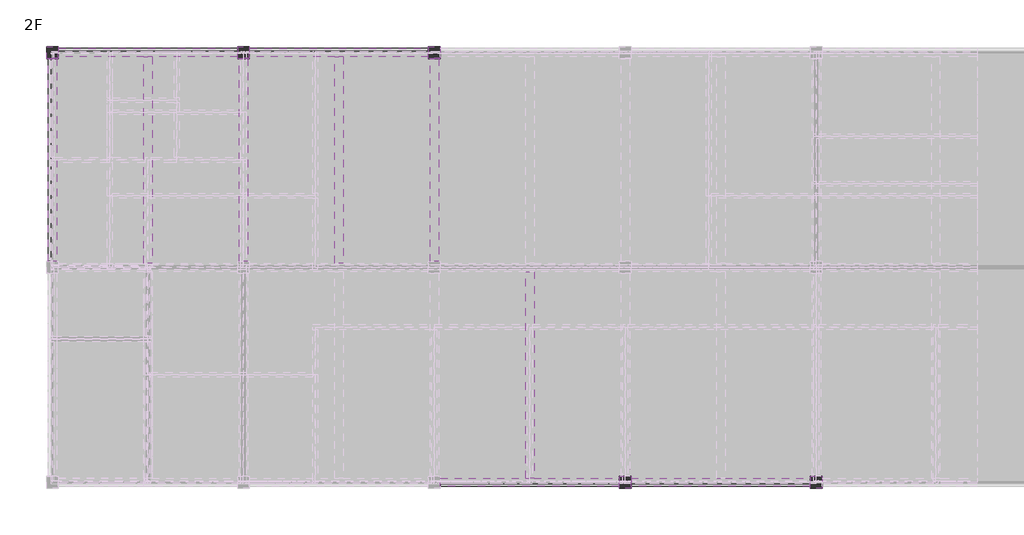
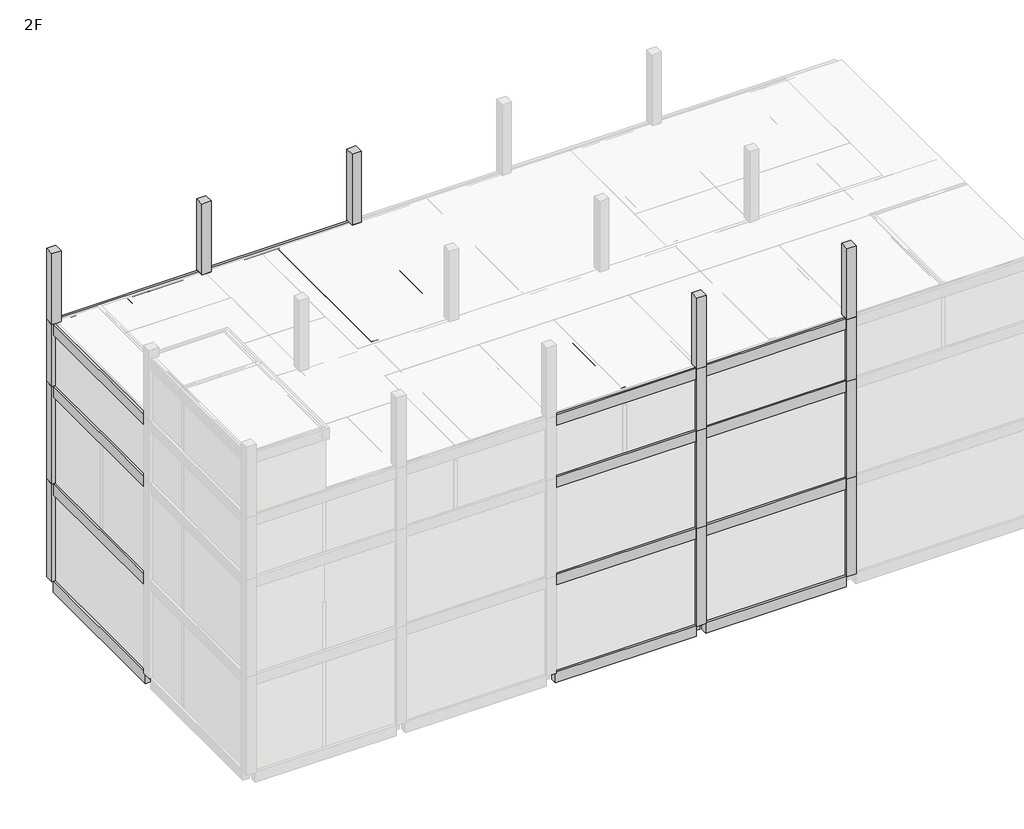
# One storey, part 5 of 7: 42 beams, 20 columns.
"""IFC4 building model written with IfcOpenShell, lengths in millimetres."""

from ifc_helpers import new_model, si_unit, frame, origin, place, context, project, spatial, polyline, outline, extrude, faceted_brep, element, save

model = new_model("IFC4")

# Units and contexts
model_context = context("Model", 3, world=origin())
ifc_project = project(units=[si_unit("LENGTHUNIT", "METRE", prefix="MILLI")], contexts=[model_context])

# Site, building, storey
site = spatial("IfcSite", under=ifc_project)
building = spatial("IfcBuilding", under=site)
storey = spatial("IfcBuildingStorey", under=building, Name="2F", Elevation=3500.0)

# Beams
placement = place(None, origin())
element("IfcBeam", 1, ObjectType="Concrete-Rectangular-Beam : BM111_400x500_RG1", at=placement, inside=storey, context=model_context, shape_type="SweptSolid", body=[
    extrude(outline(polyline([(49284.6521483, 181748.8614395), (49634.6521483, 181748.8614395), (49634.6521483, 173098.8614395), (49284.6521483, 173098.8614395), (49284.6521483, 181748.8614395)])), frame((0.0, 0.0, 2900.0), z_axis=(0.0, 0.0, 1.0), x_axis=(1.0, 0.0, 0.0)), (0.0, 0.0, 1.0), 600.0),
])
element("IfcBeam", 2, ObjectType="Concrete-Rectangular-Beam : BM111_400x500_RG1", at=placement, inside=storey, context=model_context, shape_type="SweptSolid", body=[
    extrude(outline(polyline([(57634.6521483, 173098.8614395), (57284.6521483, 173098.8614395), (57284.6521483, 181748.8614395), (57634.6521483, 181748.8614395), (57634.6521483, 173098.8614395)])), frame((0.0, 0.0, 2900.0), z_axis=(0.0, 0.0, 1.0), x_axis=(1.0, 0.0, 0.0)), (0.0, 0.0, 1.0), 600.0),
])
element("IfcBeam", 3, ObjectType="Concrete-Rectangular-Beam : BM111_400x500_RG1", at=placement, inside=storey, context=model_context, shape_type="SweptSolid", body=[
    extrude(outline(polyline([(65284.6521483, 172748.8614395), (65634.6521483, 172748.8614395), (65634.6521483, 164098.8614395), (65284.6521483, 164098.8614395), (65284.6521483, 172748.8614395)])), frame((0.0, 0.0, 2900.0), z_axis=(0.0, 0.0, 1.0), x_axis=(1.0, 0.0, 0.0)), (0.0, 0.0, 1.0), 600.0),
])
element("IfcBeam", 4, ObjectType="Concrete-Rectangular-Beam : BM111_400x500_RG1", at=placement, inside=storey, context=model_context, shape_type="SweptSolid", body=[
    extrude(outline(polyline([(49284.6521483, 181748.8614395), (49634.6521483, 181748.8614395), (49634.6521483, 173098.8614395), (49284.6521483, 173098.8614395), (49284.6521483, 181748.8614395)])), frame((0.0, 0.0, 8400.0), z_axis=(0.0, 0.0, 1.0), x_axis=(1.0, 0.0, 0.0)), (0.0, 0.0, 1.0), 600.0),
])
element("IfcBeam", 5, ObjectType="Concrete-Rectangular-Beam : BM111_400x500_RG1", at=placement, inside=storey, context=model_context, shape_type="SweptSolid", body=[
    extrude(outline(polyline([(57634.6521483, 173098.8614395), (57284.6521483, 173098.8614395), (57284.6521483, 181748.8614395), (57634.6521483, 181748.8614395), (57634.6521483, 173098.8614395)])), frame((0.0, 0.0, 8400.0), z_axis=(0.0, 0.0, 1.0), x_axis=(1.0, 0.0, 0.0)), (0.0, 0.0, 1.0), 600.0),
])
element("IfcBeam", 6, ObjectType="Concrete-Rectangular-Beam : BM111_400x500_RG1", at=placement, inside=storey, context=model_context, shape_type="SweptSolid", body=[
    extrude(outline(polyline([(65284.6521483, 172748.8614395), (65634.6521483, 172748.8614395), (65634.6521483, 164098.8614395), (65284.6521483, 164098.8614395), (65284.6521483, 172748.8614395)])), frame((0.0, 0.0, 8400.0), z_axis=(0.0, 0.0, 1.0), x_axis=(1.0, 0.0, 0.0)), (0.0, 0.0, 1.0), 600.0),
])
element("IfcBeam", 7, ObjectType="Concrete-Rectangular-Beam : BM111_400x500_RG1", at=placement, inside=storey, context=model_context, shape_type="SweptSolid", body=[
    extrude(outline(polyline([(49284.6521483, 181748.8614395), (49634.6521483, 181748.8614395), (49634.6521483, 173098.8614395), (49284.6521483, 173098.8614395), (49284.6521483, 181748.8614395)])), frame((0.0, 0.0, 13900.0), z_axis=(0.0, 0.0, 1.0), x_axis=(1.0, 0.0, 0.0)), (0.0, 0.0, 1.0), 600.0),
])
element("IfcBeam", 8, ObjectType="Concrete-Rectangular-Beam : BM111_400x500_RG1", at=placement, inside=storey, context=model_context, shape_type="SweptSolid", body=[
    extrude(outline(polyline([(57634.6521483, 173098.8614395), (57284.6521483, 173098.8614395), (57284.6521483, 181748.8614395), (57634.6521483, 181748.8614395), (57634.6521483, 173098.8614395)])), frame((0.0, 0.0, 13900.0), z_axis=(0.0, 0.0, 1.0), x_axis=(1.0, 0.0, 0.0)), (0.0, 0.0, 1.0), 600.0),
])
element("IfcBeam", 9, ObjectType="Concrete-Rectangular-Beam : BM111_400x500_RG1", at=placement, inside=storey, context=model_context, shape_type="SweptSolid", body=[
    extrude(outline(polyline([(65284.6521483, 172748.8614395), (65634.6521483, 172748.8614395), (65634.6521483, 164098.8614395), (65284.6521483, 164098.8614395), (65284.6521483, 172748.8614395)])), frame((0.0, 0.0, 13900.0), z_axis=(0.0, 0.0, 1.0), x_axis=(1.0, 0.0, 0.0)), (0.0, 0.0, 1.0), 600.0),
])
element("IfcBeam", 10, ObjectType="Concrete-Rectangular-Beam : BM111_400x500_RG1", at=placement, inside=storey, context=model_context, shape_type="SweptSolid", body=[
    extrude(outline(polyline([(49284.6521483, 181748.8614395), (49634.6521483, 181748.8614395), (49634.6521483, 173098.8614395), (49284.6521483, 173098.8614395), (49284.6521483, 181748.8614395)])), frame((0.0, 0.0, 17400.0), z_axis=(0.0, 0.0, 1.0), x_axis=(1.0, 0.0, 0.0)), (0.0, 0.0, 1.0), 600.0),
])
element("IfcBeam", 11, ObjectType="Concrete-Rectangular-Beam : BM111_400x500_RG1", at=placement, inside=storey, context=model_context, shape_type="SweptSolid", body=[
    extrude(outline(polyline([(57634.6521483, 173098.8614395), (57284.6521483, 173098.8614395), (57284.6521483, 181748.8614395), (57634.6521483, 181748.8614395), (57634.6521483, 173098.8614395)])), frame((0.0, 0.0, 17400.0), z_axis=(0.0, 0.0, 1.0), x_axis=(1.0, 0.0, 0.0)), (0.0, 0.0, 1.0), 600.0),
])
element("IfcBeam", 12, ObjectType="Concrete-Rectangular-Beam : BM111_400x500_RG1", at=placement, inside=storey, context=model_context, shape_type="SweptSolid", body=[
    extrude(outline(polyline([(65284.6521483, 172748.8614395), (65634.6521483, 172748.8614395), (65634.6521483, 164098.8614395), (65284.6521483, 164098.8614395), (65284.6521483, 172748.8614395)])), frame((0.0, 0.0, 17400.0), z_axis=(0.0, 0.0, 1.0), x_axis=(1.0, 0.0, 0.0)), (0.0, 0.0, 1.0), 600.0),
])
element("IfcBeam", 13, ObjectType="Concrete-Rectangular-Beam : BM111_400x500_RG1", at=placement, inside=storey, context=model_context, shape_type="Brep", body=[
    faceted_brep([(45709.6521483, 182098.8614395, 3500.0), (45709.6521483, 181748.8614395, 3500.0), (49284.6521483, 181748.8614395, 3500.0), (49634.6521483, 181748.8614395, 3500.0), (53209.6521483, 181748.8614395, 3500.0), (53209.6521483, 182098.8614395, 3500.0), (45709.6521483, 181748.8614395, 2900.0), (49284.6521483, 181748.8614395, 2900.0), (49634.6521483, 181748.8614395, 2900.0), (53209.6521483, 181748.8614395, 2900.0), (45709.6521483, 182098.8614395, 2900.0), (53209.6521483, 182098.8614395, 2900.0)], [[[0, 1, 2, 3, 4, 5]], [[1, 6, 7, 8, 9, 4, 3, 2]], [[6, 10, 11, 9, 8, 7]], [[10, 0, 5, 11]], [[1, 0, 10, 6]], [[5, 4, 9, 11]]]),
])
element("IfcBeam", 14, ObjectType="Concrete-Rectangular-Beam : BM111_400x500_RG1", at=placement, inside=storey, context=model_context, shape_type="Brep", body=[
    faceted_brep([(53709.6521483, 182098.8614395, 3500.0), (53709.6521483, 181748.8614395, 3500.0), (57284.6521483, 181748.8614395, 3500.0), (57634.6521483, 181748.8614395, 3500.0), (61209.6521483, 181748.8614395, 3500.0), (61209.6521483, 182098.8614395, 3500.0), (53709.6521483, 181748.8614395, 2900.0), (57284.6521483, 181748.8614395, 2900.0), (57634.6521483, 181748.8614395, 2900.0), (61209.6521483, 181748.8614395, 2900.0), (53709.6521483, 182098.8614395, 2900.0), (61209.6521483, 182098.8614395, 2900.0)], [[[0, 1, 2, 3, 4, 5]], [[1, 6, 7, 8, 9, 4, 3, 2]], [[6, 10, 11, 9, 8, 7]], [[10, 0, 5, 11]], [[1, 0, 10, 6]], [[5, 4, 9, 11]]]),
])
element("IfcBeam", 15, ObjectType="Concrete-Rectangular-Beam : BM111_400x500_RG1", at=placement, inside=storey, context=model_context, shape_type="Brep", body=[
    faceted_brep([(61709.6521483, 164098.8614395, 3500.0), (61709.6521483, 163748.8614395, 3500.0), (69209.6521483, 163748.8614395, 3500.0), (69209.6521483, 164098.8614395, 3500.0), (65634.6521483, 164098.8614395, 3500.0), (65284.6521483, 164098.8614395, 3500.0), (61709.6521483, 163748.8614395, 2900.0), (69209.6521483, 163748.8614395, 2900.0), (61709.6521483, 164098.8614395, 2900.0), (65284.6521483, 164098.8614395, 2900.0), (65634.6521483, 164098.8614395, 2900.0), (69209.6521483, 164098.8614395, 2900.0)], [[[0, 1, 2, 3, 4, 5]], [[1, 6, 7, 2]], [[6, 8, 9, 10, 11, 7]], [[8, 0, 5, 4, 3, 11, 10, 9]], [[1, 0, 8, 6]], [[3, 2, 7, 11]]]),
])
element("IfcBeam", 16, ObjectType="Concrete-Rectangular-Beam : BM111_400x500_RG1", at=placement, inside=storey, context=model_context, shape_type="Brep", body=[
    faceted_brep([(69709.6521483, 164098.8614395, 3500.0), (69709.6521483, 163748.8614395, 3500.0), (77209.6521483, 163748.8614395, 3500.0), (77209.6521483, 164098.8614395, 3500.0), (73634.6521483, 164098.8614395, 3500.0), (73284.6521483, 164098.8614395, 3500.0), (69709.6521483, 163748.8614395, 2900.0), (77209.6521483, 163748.8614395, 2900.0), (69709.6521483, 164098.8614395, 2900.0), (73284.6521483, 164098.8614395, 2900.0), (73634.6521483, 164098.8614395, 2900.0), (77209.6521483, 164098.8614395, 2900.0)], [[[0, 1, 2, 3, 4, 5]], [[1, 6, 7, 2]], [[6, 8, 9, 10, 11, 7]], [[8, 0, 5, 4, 3, 11, 10, 9]], [[1, 0, 8, 6]], [[3, 2, 7, 11]]]),
])
element("IfcBeam", 17, ObjectType="Concrete-Rectangular-Beam : BM111_400x500_RG1", at=placement, inside=storey, context=model_context, shape_type="Brep", body=[
    faceted_brep([(45709.6521483, 182098.8614395, 9000.0), (45709.6521483, 181748.8614395, 9000.0), (49284.6521483, 181748.8614395, 9000.0), (49634.6521483, 181748.8614395, 9000.0), (53209.6521483, 181748.8614395, 9000.0), (53209.6521483, 182098.8614395, 9000.0), (45709.6521483, 181748.8614395, 8400.0), (49284.6521483, 181748.8614395, 8400.0), (49634.6521483, 181748.8614395, 8400.0), (53209.6521483, 181748.8614395, 8400.0), (45709.6521483, 182098.8614395, 8400.0), (53209.6521483, 182098.8614395, 8400.0)], [[[0, 1, 2, 3, 4, 5]], [[1, 6, 7, 8, 9, 4, 3, 2]], [[6, 10, 11, 9, 8, 7]], [[10, 0, 5, 11]], [[1, 0, 10, 6]], [[5, 4, 9, 11]]]),
])
element("IfcBeam", 18, ObjectType="Concrete-Rectangular-Beam : BM111_400x500_RG1", at=placement, inside=storey, context=model_context, shape_type="Brep", body=[
    faceted_brep([(53709.6521483, 182098.8614395, 9000.0), (53709.6521483, 181748.8614395, 9000.0), (57284.6521483, 181748.8614395, 9000.0), (57634.6521483, 181748.8614395, 9000.0), (61209.6521483, 181748.8614395, 9000.0), (61209.6521483, 182098.8614395, 9000.0), (53709.6521483, 181748.8614395, 8400.0), (57284.6521483, 181748.8614395, 8400.0), (57634.6521483, 181748.8614395, 8400.0), (61209.6521483, 181748.8614395, 8400.0), (53709.6521483, 182098.8614395, 8400.0), (61209.6521483, 182098.8614395, 8400.0)], [[[0, 1, 2, 3, 4, 5]], [[1, 6, 7, 8, 9, 4, 3, 2]], [[6, 10, 11, 9, 8, 7]], [[10, 0, 5, 11]], [[1, 0, 10, 6]], [[5, 4, 9, 11]]]),
])
element("IfcBeam", 19, ObjectType="Concrete-Rectangular-Beam : BM111_400x500_RG1", at=placement, inside=storey, context=model_context, shape_type="Brep", body=[
    faceted_brep([(61709.6521483, 164098.8614395, 9000.0), (61709.6521483, 163748.8614395, 9000.0), (69209.6521483, 163748.8614395, 9000.0), (69209.6521483, 164098.8614395, 9000.0), (65634.6521483, 164098.8614395, 9000.0), (65284.6521483, 164098.8614395, 9000.0), (61709.6521483, 163748.8614395, 8400.0), (69209.6521483, 163748.8614395, 8400.0), (61709.6521483, 164098.8614395, 8400.0), (65284.6521483, 164098.8614395, 8400.0), (65634.6521483, 164098.8614395, 8400.0), (69209.6521483, 164098.8614395, 8400.0)], [[[0, 1, 2, 3, 4, 5]], [[1, 6, 7, 2]], [[6, 8, 9, 10, 11, 7]], [[8, 0, 5, 4, 3, 11, 10, 9]], [[1, 0, 8, 6]], [[3, 2, 7, 11]]]),
])
element("IfcBeam", 20, ObjectType="Concrete-Rectangular-Beam : BM111_400x500_RG1", at=placement, inside=storey, context=model_context, shape_type="Brep", body=[
    faceted_brep([(69709.6521483, 164098.8614395, 9000.0), (69709.6521483, 163748.8614395, 9000.0), (77209.6521483, 163748.8614395, 9000.0), (77209.6521483, 164098.8614395, 9000.0), (73634.6521483, 164098.8614395, 9000.0), (73284.6521483, 164098.8614395, 9000.0), (69709.6521483, 163748.8614395, 8400.0), (77209.6521483, 163748.8614395, 8400.0), (69709.6521483, 164098.8614395, 8400.0), (73284.6521483, 164098.8614395, 8400.0), (73634.6521483, 164098.8614395, 8400.0), (77209.6521483, 164098.8614395, 8400.0)], [[[0, 1, 2, 3, 4, 5]], [[1, 6, 7, 2]], [[6, 8, 9, 10, 11, 7]], [[8, 0, 5, 4, 3, 11, 10, 9]], [[1, 0, 8, 6]], [[3, 2, 7, 11]]]),
])
element("IfcBeam", 21, ObjectType="Concrete-Rectangular-Beam : BM111_400x500_RG1", at=placement, inside=storey, context=model_context, shape_type="Brep", body=[
    faceted_brep([(45709.6521483, 182098.8614395, 14500.0), (45709.6521483, 181748.8614395, 14500.0), (49284.6521483, 181748.8614395, 14500.0), (49634.6521483, 181748.8614395, 14500.0), (53209.6521483, 181748.8614395, 14500.0), (53209.6521483, 182098.8614395, 14500.0), (45709.6521483, 181748.8614395, 13900.0), (49284.6521483, 181748.8614395, 13900.0), (49634.6521483, 181748.8614395, 13900.0), (53209.6521483, 181748.8614395, 13900.0), (45709.6521483, 182098.8614395, 13900.0), (53209.6521483, 182098.8614395, 13900.0)], [[[0, 1, 2, 3, 4, 5]], [[1, 6, 7, 8, 9, 4, 3, 2]], [[6, 10, 11, 9, 8, 7]], [[10, 0, 5, 11]], [[1, 0, 10, 6]], [[5, 4, 9, 11]]]),
])
element("IfcBeam", 22, ObjectType="Concrete-Rectangular-Beam : BM111_400x500_RG1", at=placement, inside=storey, context=model_context, shape_type="Brep", body=[
    faceted_brep([(53709.6521483, 182098.8614395, 14500.0), (53709.6521483, 181748.8614395, 14500.0), (57284.6521483, 181748.8614395, 14500.0), (57634.6521483, 181748.8614395, 14500.0), (61209.6521483, 181748.8614395, 14500.0), (61209.6521483, 182098.8614395, 14500.0), (53709.6521483, 181748.8614395, 13900.0), (57284.6521483, 181748.8614395, 13900.0), (57634.6521483, 181748.8614395, 13900.0), (61209.6521483, 181748.8614395, 13900.0), (53709.6521483, 182098.8614395, 13900.0), (61209.6521483, 182098.8614395, 13900.0)], [[[0, 1, 2, 3, 4, 5]], [[1, 6, 7, 8, 9, 4, 3, 2]], [[6, 10, 11, 9, 8, 7]], [[10, 0, 5, 11]], [[1, 0, 10, 6]], [[5, 4, 9, 11]]]),
])
element("IfcBeam", 23, ObjectType="Concrete-Rectangular-Beam : BM111_400x500_RG1", at=placement, inside=storey, context=model_context, shape_type="Brep", body=[
    faceted_brep([(61709.6521483, 164098.8614395, 14500.0), (61709.6521483, 163748.8614395, 14500.0), (69209.6521483, 163748.8614395, 14500.0), (69209.6521483, 164098.8614395, 14500.0), (65634.6521483, 164098.8614395, 14500.0), (65284.6521483, 164098.8614395, 14500.0), (61709.6521483, 163748.8614395, 13900.0), (69209.6521483, 163748.8614395, 13900.0), (61709.6521483, 164098.8614395, 13900.0), (65284.6521483, 164098.8614395, 13900.0), (65634.6521483, 164098.8614395, 13900.0), (69209.6521483, 164098.8614395, 13900.0)], [[[0, 1, 2, 3, 4, 5]], [[1, 6, 7, 2]], [[6, 8, 9, 10, 11, 7]], [[8, 0, 5, 4, 3, 11, 10, 9]], [[1, 0, 8, 6]], [[3, 2, 7, 11]]]),
])
element("IfcBeam", 24, ObjectType="Concrete-Rectangular-Beam : BM111_400x500_RG1", at=placement, inside=storey, context=model_context, shape_type="Brep", body=[
    faceted_brep([(69709.6521483, 164098.8614395, 14500.0), (69709.6521483, 163748.8614395, 14500.0), (77209.6521483, 163748.8614395, 14500.0), (77209.6521483, 164098.8614395, 14500.0), (73634.6521483, 164098.8614395, 14500.0), (73284.6521483, 164098.8614395, 14500.0), (69709.6521483, 163748.8614395, 13900.0), (77209.6521483, 163748.8614395, 13900.0), (69709.6521483, 164098.8614395, 13900.0), (73284.6521483, 164098.8614395, 13900.0), (73634.6521483, 164098.8614395, 13900.0), (77209.6521483, 164098.8614395, 13900.0)], [[[0, 1, 2, 3, 4, 5]], [[1, 6, 7, 2]], [[6, 8, 9, 10, 11, 7]], [[8, 0, 5, 4, 3, 11, 10, 9]], [[1, 0, 8, 6]], [[3, 2, 7, 11]]]),
])
element("IfcBeam", 25, ObjectType="Concrete-Rectangular-Beam : BM111_400x500_RG1", at=placement, inside=storey, context=model_context, shape_type="Brep", body=[
    faceted_brep([(45709.6521483, 182098.8614395, 18000.0), (45709.6521483, 181748.8614395, 18000.0), (49284.6521483, 181748.8614395, 18000.0), (49634.6521483, 181748.8614395, 18000.0), (53209.6521483, 181748.8614395, 18000.0), (53209.6521483, 182098.8614395, 18000.0), (45709.6521483, 181748.8614395, 17400.0), (49284.6521483, 181748.8614395, 17400.0), (49634.6521483, 181748.8614395, 17400.0), (53209.6521483, 181748.8614395, 17400.0), (45709.6521483, 182098.8614395, 17400.0), (53209.6521483, 182098.8614395, 17400.0)], [[[0, 1, 2, 3, 4, 5]], [[1, 6, 7, 8, 9, 4, 3, 2]], [[6, 10, 11, 9, 8, 7]], [[10, 0, 5, 11]], [[1, 0, 10, 6]], [[5, 4, 9, 11]]]),
])
element("IfcBeam", 26, ObjectType="Concrete-Rectangular-Beam : BM111_400x500_RG1", at=placement, inside=storey, context=model_context, shape_type="Brep", body=[
    faceted_brep([(53709.6521483, 182098.8614395, 18000.0), (53709.6521483, 181748.8614395, 18000.0), (57284.6521483, 181748.8614395, 18000.0), (57634.6521483, 181748.8614395, 18000.0), (61209.6521483, 181748.8614395, 18000.0), (61209.6521483, 182098.8614395, 18000.0), (53709.6521483, 181748.8614395, 17400.0), (57284.6521483, 181748.8614395, 17400.0), (57634.6521483, 181748.8614395, 17400.0), (61209.6521483, 181748.8614395, 17400.0), (53709.6521483, 182098.8614395, 17400.0), (61209.6521483, 182098.8614395, 17400.0)], [[[0, 1, 2, 3, 4, 5]], [[1, 6, 7, 8, 9, 4, 3, 2]], [[6, 10, 11, 9, 8, 7]], [[10, 0, 5, 11]], [[1, 0, 10, 6]], [[5, 4, 9, 11]]]),
])
element("IfcBeam", 27, ObjectType="Concrete-Rectangular-Beam : BM111_400x500_RG1", at=placement, inside=storey, context=model_context, shape_type="Brep", body=[
    faceted_brep([(61709.6521483, 164098.8614395, 18000.0), (61709.6521483, 163748.8614395, 18000.0), (69209.6521483, 163748.8614395, 18000.0), (69209.6521483, 164098.8614395, 18000.0), (65634.6521483, 164098.8614395, 18000.0), (65284.6521483, 164098.8614395, 18000.0), (61709.6521483, 163748.8614395, 17400.0), (69209.6521483, 163748.8614395, 17400.0), (61709.6521483, 164098.8614395, 17400.0), (65284.6521483, 164098.8614395, 17400.0), (65634.6521483, 164098.8614395, 17400.0), (69209.6521483, 164098.8614395, 17400.0)], [[[0, 1, 2, 3, 4, 5]], [[1, 6, 7, 2]], [[6, 8, 9, 10, 11, 7]], [[8, 0, 5, 4, 3, 11, 10, 9]], [[1, 0, 8, 6]], [[3, 2, 7, 11]]]),
])
element("IfcBeam", 28, ObjectType="Concrete-Rectangular-Beam : BM111_400x500_RG1", at=placement, inside=storey, context=model_context, shape_type="Brep", body=[
    faceted_brep([(69709.6521483, 164098.8614395, 18000.0), (69709.6521483, 163748.8614395, 18000.0), (77209.6521483, 163748.8614395, 18000.0), (77209.6521483, 164098.8614395, 18000.0), (73634.6521483, 164098.8614395, 18000.0), (73284.6521483, 164098.8614395, 18000.0), (69709.6521483, 163748.8614395, 17400.0), (77209.6521483, 163748.8614395, 17400.0), (69709.6521483, 164098.8614395, 17400.0), (73284.6521483, 164098.8614395, 17400.0), (73634.6521483, 164098.8614395, 17400.0), (77209.6521483, 164098.8614395, 17400.0)], [[[0, 1, 2, 3, 4, 5]], [[1, 6, 7, 2]], [[6, 8, 9, 10, 11, 7]], [[8, 0, 5, 4, 3, 11, 10, 9]], [[1, 0, 8, 6]], [[3, 2, 7, 11]]]),
])
element("IfcBeam", 29, ObjectType="Concrete-Rectangular-Beam : BM111_400x500_RG1", at=placement, inside=storey, context=model_context, shape_type="SweptSolid", body=[
    extrude(outline(polyline([(45284.6521483, 181673.8614395), (45634.6521483, 181673.8614395), (45634.6521483, 173173.8614395), (45284.6521483, 173173.8614395), (45284.6521483, 181673.8614395)])), frame((0.0, 0.0, 2900.0), z_axis=(0.0, 0.0, 1.0), x_axis=(1.0, 0.0, 0.0)), (0.0, 0.0, 1.0), 600.0),
])
element("IfcBeam", 30, ObjectType="Concrete-Rectangular-Beam : BM111_400x500_RG1", at=placement, inside=storey, context=model_context, shape_type="SweptSolid", body=[
    extrude(outline(polyline([(53284.6521483, 181673.8614395), (53634.6521483, 181673.8614395), (53634.6521483, 173173.8614395), (53284.6521483, 173173.8614395), (53284.6521483, 181673.8614395)])), frame((0.0, 0.0, 2900.0), z_axis=(0.0, 0.0, 1.0), x_axis=(1.0, 0.0, 0.0)), (0.0, 0.0, 1.0), 600.0),
])
element("IfcBeam", 31, ObjectType="Concrete-Rectangular-Beam : BM111_400x500_RG1", at=placement, inside=storey, context=model_context, shape_type="SweptSolid", body=[
    extrude(outline(polyline([(61284.6521483, 181673.8614395), (61634.6521483, 181673.8614395), (61634.6521483, 173173.8614395), (61284.6521483, 173173.8614395), (61284.6521483, 181673.8614395)])), frame((0.0, 0.0, 2900.0), z_axis=(0.0, 0.0, 1.0), x_axis=(1.0, 0.0, 0.0)), (0.0, 0.0, 1.0), 600.0),
])
element("IfcBeam", 32, ObjectType="Concrete-Rectangular-Beam : BM111_400x500_RG1", at=placement, inside=storey, context=model_context, shape_type="SweptSolid", body=[
    extrude(outline(polyline([(69284.6521483, 172673.8614395), (69634.6521483, 172673.8614395), (69634.6521483, 164173.8614395), (69284.6521483, 164173.8614395), (69284.6521483, 172673.8614395)])), frame((0.0, 0.0, 2900.0), z_axis=(0.0, 0.0, 1.0), x_axis=(1.0, 0.0, 0.0)), (0.0, 0.0, 1.0), 600.0),
])
element("IfcBeam", 33, ObjectType="Concrete-Rectangular-Beam : BM111_400x500_RG1", at=placement, inside=storey, context=model_context, shape_type="SweptSolid", body=[
    extrude(outline(polyline([(45284.6521483, 181673.8614395), (45634.6521483, 181673.8614395), (45634.6521483, 173173.8614395), (45284.6521483, 173173.8614395), (45284.6521483, 181673.8614395)])), frame((0.0, 0.0, 8400.0), z_axis=(0.0, 0.0, 1.0), x_axis=(1.0, 0.0, 0.0)), (0.0, 0.0, 1.0), 600.0),
])
element("IfcBeam", 34, ObjectType="Concrete-Rectangular-Beam : BM111_400x500_RG1", at=placement, inside=storey, context=model_context, shape_type="SweptSolid", body=[
    extrude(outline(polyline([(53284.6521483, 181673.8614395), (53634.6521483, 181673.8614395), (53634.6521483, 173173.8614395), (53284.6521483, 173173.8614395), (53284.6521483, 181673.8614395)])), frame((0.0, 0.0, 8400.0), z_axis=(0.0, 0.0, 1.0), x_axis=(1.0, 0.0, 0.0)), (0.0, 0.0, 1.0), 600.0),
])
element("IfcBeam", 35, ObjectType="Concrete-Rectangular-Beam : BM111_400x500_RG1", at=placement, inside=storey, context=model_context, shape_type="SweptSolid", body=[
    extrude(outline(polyline([(61284.6521483, 181673.8614395), (61634.6521483, 181673.8614395), (61634.6521483, 173173.8614395), (61284.6521483, 173173.8614395), (61284.6521483, 181673.8614395)])), frame((0.0, 0.0, 8400.0), z_axis=(0.0, 0.0, 1.0), x_axis=(1.0, 0.0, 0.0)), (0.0, 0.0, 1.0), 600.0),
])
element("IfcBeam", 36, ObjectType="Concrete-Rectangular-Beam : BM111_400x500_RG1", at=placement, inside=storey, context=model_context, shape_type="SweptSolid", body=[
    extrude(outline(polyline([(69284.6521483, 172673.8614395), (69634.6521483, 172673.8614395), (69634.6521483, 164173.8614395), (69284.6521483, 164173.8614395), (69284.6521483, 172673.8614395)])), frame((0.0, 0.0, 8400.0), z_axis=(0.0, 0.0, 1.0), x_axis=(1.0, 0.0, 0.0)), (0.0, 0.0, 1.0), 600.0),
])
element("IfcBeam", 37, ObjectType="Concrete-Rectangular-Beam : BM111_400x500_RG1", at=placement, inside=storey, context=model_context, shape_type="SweptSolid", body=[
    extrude(outline(polyline([(45284.6521483, 181673.8614395), (45634.6521483, 181673.8614395), (45634.6521483, 173173.8614395), (45284.6521483, 173173.8614395), (45284.6521483, 181673.8614395)])), frame((0.0, 0.0, 13900.0), z_axis=(0.0, 0.0, 1.0), x_axis=(1.0, 0.0, 0.0)), (0.0, 0.0, 1.0), 600.0),
])
element("IfcBeam", 38, ObjectType="Concrete-Rectangular-Beam : BM111_400x500_RG1", at=placement, inside=storey, context=model_context, shape_type="SweptSolid", body=[
    extrude(outline(polyline([(53284.6521483, 181673.8614395), (53634.6521483, 181673.8614395), (53634.6521483, 173173.8614395), (53284.6521483, 173173.8614395), (53284.6521483, 181673.8614395)])), frame((0.0, 0.0, 13900.0), z_axis=(0.0, 0.0, 1.0), x_axis=(1.0, 0.0, 0.0)), (0.0, 0.0, 1.0), 600.0),
])
element("IfcBeam", 39, ObjectType="Concrete-Rectangular-Beam : BM111_400x500_RG1", at=placement, inside=storey, context=model_context, shape_type="SweptSolid", body=[
    extrude(outline(polyline([(61284.6521483, 181673.8614395), (61634.6521483, 181673.8614395), (61634.6521483, 173173.8614395), (61284.6521483, 173173.8614395), (61284.6521483, 181673.8614395)])), frame((0.0, 0.0, 13900.0), z_axis=(0.0, 0.0, 1.0), x_axis=(1.0, 0.0, 0.0)), (0.0, 0.0, 1.0), 600.0),
])
element("IfcBeam", 40, ObjectType="Concrete-Rectangular-Beam : BM111_400x500_RG1", at=placement, inside=storey, context=model_context, shape_type="SweptSolid", body=[
    extrude(outline(polyline([(45284.6521483, 181673.8614395), (45634.6521483, 181673.8614395), (45634.6521483, 173173.8614395), (45284.6521483, 173173.8614395), (45284.6521483, 181673.8614395)])), frame((0.0, 0.0, 17400.0), z_axis=(0.0, 0.0, 1.0), x_axis=(1.0, 0.0, 0.0)), (0.0, 0.0, 1.0), 600.0),
])
element("IfcBeam", 41, ObjectType="Concrete-Rectangular-Beam : BM111_400x500_RG1", at=placement, inside=storey, context=model_context, shape_type="SweptSolid", body=[
    extrude(outline(polyline([(53284.6521483, 181673.8614395), (53634.6521483, 181673.8614395), (53634.6521483, 173173.8614395), (53284.6521483, 173173.8614395), (53284.6521483, 181673.8614395)])), frame((0.0, 0.0, 17400.0), z_axis=(0.0, 0.0, 1.0), x_axis=(1.0, 0.0, 0.0)), (0.0, 0.0, 1.0), 600.0),
])
element("IfcBeam", 42, ObjectType="Concrete-Rectangular-Beam : BM111_400x500_RG1", at=placement, inside=storey, context=model_context, shape_type="SweptSolid", body=[
    extrude(outline(polyline([(61284.6521483, 181673.8614395), (61634.6521483, 181673.8614395), (61634.6521483, 173173.8614395), (61284.6521483, 173173.8614395), (61284.6521483, 181673.8614395)])), frame((0.0, 0.0, 17400.0), z_axis=(0.0, 0.0, 1.0), x_axis=(1.0, 0.0, 0.0)), (0.0, 0.0, 1.0), 600.0),
])

# Columns
element("IfcColumn", 43, ObjectType="Concrete-Rectangular-Column : CL111_500x500", at=placement, inside=storey, context=model_context, shape_type="Brep", body=[
    faceted_brep([(45709.6521483, 182173.8614395, 3500.0), (45709.6521483, 181673.8614395, 3500.0), (45209.6521483, 181673.8614395, 3500.0), (45209.6521483, 182173.8614395, 3500.0), (45709.6521483, 182173.8614395, 9000.0), (45709.6521483, 182098.8614395, 9000.0), (45709.6521483, 181748.8614395, 9000.0), (45709.6521483, 181673.8614395, 9000.0), (45634.6521483, 181673.8614395, 9000.0), (45284.6521483, 181673.8614395, 9000.0), (45209.6521483, 181673.8614395, 9000.0), (45209.6521483, 182173.8614395, 9000.0)], [[[0, 1, 2, 3]], [[4, 5, 6, 7, 1, 0]], [[7, 8, 9, 10, 2, 1]], [[10, 11, 3, 2]], [[11, 4, 0, 3]], [[4, 11, 10, 9, 8, 7, 6, 5]]]),
])
element("IfcColumn", 44, ObjectType="Concrete-Rectangular-Column : CL111_500x500", at=placement, inside=storey, context=model_context, shape_type="Brep", body=[
    faceted_brep([(45709.6521483, 182173.8614395, 9000.0), (45709.6521483, 181673.8614395, 9000.0), (45209.6521483, 181673.8614395, 9000.0), (45209.6521483, 182173.8614395, 9000.0), (45709.6521483, 182173.8614395, 14500.0), (45709.6521483, 182098.8614395, 14500.0), (45709.6521483, 181748.8614395, 14500.0), (45709.6521483, 181673.8614395, 14500.0), (45634.6521483, 181673.8614395, 14500.0), (45284.6521483, 181673.8614395, 14500.0), (45209.6521483, 181673.8614395, 14500.0), (45209.6521483, 182173.8614395, 14500.0)], [[[0, 1, 2, 3]], [[4, 5, 6, 7, 1, 0]], [[7, 8, 9, 10, 2, 1]], [[10, 11, 3, 2]], [[11, 4, 0, 3]], [[4, 11, 10, 9, 8, 7, 6, 5]]]),
])
element("IfcColumn", 45, ObjectType="Concrete-Rectangular-Column : CL111_500x500", at=placement, inside=storey, context=model_context, shape_type="Brep", body=[
    faceted_brep([(45709.6521483, 182173.8614395, 14500.0), (45709.6521483, 181673.8614395, 14500.0), (45209.6521483, 181673.8614395, 14500.0), (45209.6521483, 182173.8614395, 14500.0), (45709.6521483, 182173.8614395, 18000.0), (45709.6521483, 182098.8614395, 18000.0), (45709.6521483, 181748.8614395, 18000.0), (45709.6521483, 181673.8614395, 18000.0), (45634.6521483, 181673.8614395, 18000.0), (45284.6521483, 181673.8614395, 18000.0), (45209.6521483, 181673.8614395, 18000.0), (45209.6521483, 182173.8614395, 18000.0)], [[[0, 1, 2, 3]], [[4, 5, 6, 7, 1, 0]], [[7, 8, 9, 10, 2, 1]], [[10, 11, 3, 2]], [[11, 4, 0, 3]], [[4, 11, 10, 9, 8, 7, 6, 5]]]),
])
element("IfcColumn", 46, ObjectType="Concrete-Rectangular-Column : CL111_500x500", at=placement, inside=storey, context=model_context, shape_type="SweptSolid", body=[
    extrude(outline(polyline([(45709.6521483, 182173.8614395), (45709.6521483, 181673.8614395), (45209.6521483, 181673.8614395), (45209.6521483, 182173.8614395), (45709.6521483, 182173.8614395)])), frame((0.0, 0.0, 18000.0), z_axis=(0.0, 0.0, 1.0), x_axis=(1.0, 0.0, 0.0)), (0.0, 0.0, 1.0), 4000.0),
])
element("IfcColumn", 47, ObjectType="Concrete-Rectangular-Column : CL111_500x500", at=placement, inside=storey, context=model_context, shape_type="Brep", body=[
    faceted_brep([(53709.6521483, 182173.8614395, 3500.0), (53709.6521483, 181673.8614395, 3500.0), (53209.6521483, 181673.8614395, 3500.0), (53209.6521483, 182173.8614395, 3500.0), (53709.6521483, 182173.8614395, 9000.0), (53709.6521483, 182098.8614395, 9000.0), (53709.6521483, 181748.8614395, 9000.0), (53709.6521483, 181673.8614395, 9000.0), (53634.6521483, 181673.8614395, 9000.0), (53284.6521483, 181673.8614395, 9000.0), (53209.6521483, 181673.8614395, 9000.0), (53209.6521483, 181748.8614395, 9000.0), (53209.6521483, 182098.8614395, 9000.0), (53209.6521483, 182173.8614395, 9000.0)], [[[0, 1, 2, 3]], [[4, 5, 6, 7, 1, 0]], [[7, 8, 9, 10, 2, 1]], [[10, 11, 12, 13, 3, 2]], [[13, 4, 0, 3]], [[4, 13, 12, 11, 10, 9, 8, 7, 6, 5]]]),
])
element("IfcColumn", 48, ObjectType="Concrete-Rectangular-Column : CL111_500x500", at=placement, inside=storey, context=model_context, shape_type="Brep", body=[
    faceted_brep([(53709.6521483, 182173.8614395, 9000.0), (53709.6521483, 181673.8614395, 9000.0), (53209.6521483, 181673.8614395, 9000.0), (53209.6521483, 182173.8614395, 9000.0), (53709.6521483, 182173.8614395, 14500.0), (53709.6521483, 182098.8614395, 14500.0), (53709.6521483, 181748.8614395, 14500.0), (53709.6521483, 181673.8614395, 14500.0), (53634.6521483, 181673.8614395, 14500.0), (53284.6521483, 181673.8614395, 14500.0), (53209.6521483, 181673.8614395, 14500.0), (53209.6521483, 181748.8614395, 14500.0), (53209.6521483, 182098.8614395, 14500.0), (53209.6521483, 182173.8614395, 14500.0)], [[[0, 1, 2, 3]], [[4, 5, 6, 7, 1, 0]], [[7, 8, 9, 10, 2, 1]], [[10, 11, 12, 13, 3, 2]], [[13, 4, 0, 3]], [[4, 13, 12, 11, 10, 9, 8, 7, 6, 5]]]),
])
element("IfcColumn", 49, ObjectType="Concrete-Rectangular-Column : CL111_500x500", at=placement, inside=storey, context=model_context, shape_type="Brep", body=[
    faceted_brep([(53709.6521483, 182173.8614395, 14500.0), (53709.6521483, 181673.8614395, 14500.0), (53209.6521483, 181673.8614395, 14500.0), (53209.6521483, 182173.8614395, 14500.0), (53709.6521483, 182173.8614395, 18000.0), (53709.6521483, 182098.8614395, 18000.0), (53709.6521483, 181748.8614395, 18000.0), (53709.6521483, 181673.8614395, 18000.0), (53634.6521483, 181673.8614395, 18000.0), (53284.6521483, 181673.8614395, 18000.0), (53209.6521483, 181673.8614395, 18000.0), (53209.6521483, 181748.8614395, 18000.0), (53209.6521483, 182098.8614395, 18000.0), (53209.6521483, 182173.8614395, 18000.0)], [[[0, 1, 2, 3]], [[4, 5, 6, 7, 1, 0]], [[7, 8, 9, 10, 2, 1]], [[10, 11, 12, 13, 3, 2]], [[13, 4, 0, 3]], [[4, 13, 12, 11, 10, 9, 8, 7, 6, 5]]]),
])
element("IfcColumn", 50, ObjectType="Concrete-Rectangular-Column : CL111_500x500", at=placement, inside=storey, context=model_context, shape_type="SweptSolid", body=[
    extrude(outline(polyline([(53709.6521483, 182173.8614395), (53709.6521483, 181673.8614395), (53209.6521483, 181673.8614395), (53209.6521483, 182173.8614395), (53709.6521483, 182173.8614395)])), frame((0.0, 0.0, 18000.0), z_axis=(0.0, 0.0, 1.0), x_axis=(1.0, 0.0, 0.0)), (0.0, 0.0, 1.0), 4000.0),
])
element("IfcColumn", 51, ObjectType="Concrete-Rectangular-Column : CL111_500x500", at=placement, inside=storey, context=model_context, shape_type="Brep", body=[
    faceted_brep([(61709.6521483, 182173.8614395, 3500.0), (61709.6521483, 181673.8614395, 3500.0), (61209.6521483, 181673.8614395, 3500.0), (61209.6521483, 182173.8614395, 3500.0), (61709.6521483, 182173.8614395, 9000.0), (61709.6521483, 182098.8614395, 9000.0), (61709.6521483, 181748.8614395, 9000.0), (61709.6521483, 181673.8614395, 9000.0), (61634.6521483, 181673.8614395, 9000.0), (61284.6521483, 181673.8614395, 9000.0), (61209.6521483, 181673.8614395, 9000.0), (61209.6521483, 181748.8614395, 9000.0), (61209.6521483, 182098.8614395, 9000.0), (61209.6521483, 182173.8614395, 9000.0)], [[[0, 1, 2, 3]], [[4, 5, 6, 7, 1, 0]], [[7, 8, 9, 10, 2, 1]], [[10, 11, 12, 13, 3, 2]], [[13, 4, 0, 3]], [[4, 13, 12, 11, 10, 9, 8, 7, 6, 5]]]),
])
element("IfcColumn", 52, ObjectType="Concrete-Rectangular-Column : CL111_500x500", at=placement, inside=storey, context=model_context, shape_type="Brep", body=[
    faceted_brep([(61709.6521483, 182173.8614395, 9000.0), (61709.6521483, 181673.8614395, 9000.0), (61209.6521483, 181673.8614395, 9000.0), (61209.6521483, 182173.8614395, 9000.0), (61709.6521483, 182173.8614395, 14500.0), (61709.6521483, 182098.8614395, 14500.0), (61709.6521483, 181748.8614395, 14500.0), (61709.6521483, 181673.8614395, 14500.0), (61634.6521483, 181673.8614395, 14500.0), (61284.6521483, 181673.8614395, 14500.0), (61209.6521483, 181673.8614395, 14500.0), (61209.6521483, 181748.8614395, 14500.0), (61209.6521483, 182098.8614395, 14500.0), (61209.6521483, 182173.8614395, 14500.0)], [[[0, 1, 2, 3]], [[4, 5, 6, 7, 1, 0]], [[7, 8, 9, 10, 2, 1]], [[10, 11, 12, 13, 3, 2]], [[13, 4, 0, 3]], [[4, 13, 12, 11, 10, 9, 8, 7, 6, 5]]]),
])
element("IfcColumn", 53, ObjectType="Concrete-Rectangular-Column : CL111_500x500", at=placement, inside=storey, context=model_context, shape_type="Brep", body=[
    faceted_brep([(61709.6521483, 182173.8614395, 14500.0), (61709.6521483, 181673.8614395, 14500.0), (61209.6521483, 181673.8614395, 14500.0), (61209.6521483, 182173.8614395, 14500.0), (61709.6521483, 182173.8614395, 18000.0), (61709.6521483, 182098.8614395, 18000.0), (61709.6521483, 181748.8614395, 18000.0), (61709.6521483, 181673.8614395, 18000.0), (61634.6521483, 181673.8614395, 18000.0), (61284.6521483, 181673.8614395, 18000.0), (61209.6521483, 181673.8614395, 18000.0), (61209.6521483, 181748.8614395, 18000.0), (61209.6521483, 182098.8614395, 18000.0), (61209.6521483, 182173.8614395, 18000.0)], [[[0, 1, 2, 3]], [[4, 5, 6, 7, 1, 0]], [[7, 8, 9, 10, 2, 1]], [[10, 11, 12, 13, 3, 2]], [[13, 4, 0, 3]], [[4, 13, 12, 11, 10, 9, 8, 7, 6, 5]]]),
])
element("IfcColumn", 54, ObjectType="Concrete-Rectangular-Column : CL111_500x500", at=placement, inside=storey, context=model_context, shape_type="SweptSolid", body=[
    extrude(outline(polyline([(61709.6521483, 182173.8614395), (61709.6521483, 181673.8614395), (61209.6521483, 181673.8614395), (61209.6521483, 182173.8614395), (61709.6521483, 182173.8614395)])), frame((0.0, 0.0, 18000.0), z_axis=(0.0, 0.0, 1.0), x_axis=(1.0, 0.0, 0.0)), (0.0, 0.0, 1.0), 4000.0),
])
element("IfcColumn", 55, ObjectType="Concrete-Rectangular-Column : CL111_500x500", at=placement, inside=storey, context=model_context, shape_type="Brep", body=[
    faceted_brep([(69709.6521483, 164173.8614395, 3500.0), (69709.6521483, 163673.8614395, 3500.0), (69209.6521483, 163673.8614395, 3500.0), (69209.6521483, 164173.8614395, 3500.0), (69709.6521483, 164173.8614395, 9000.0), (69709.6521483, 164098.8614395, 9000.0), (69709.6521483, 163748.8614395, 9000.0), (69709.6521483, 163673.8614395, 9000.0), (69209.6521483, 163673.8614395, 9000.0), (69209.6521483, 163748.8614395, 9000.0), (69209.6521483, 164098.8614395, 9000.0), (69209.6521483, 164173.8614395, 9000.0), (69284.6521483, 164173.8614395, 9000.0), (69634.6521483, 164173.8614395, 9000.0)], [[[0, 1, 2, 3]], [[4, 5, 6, 7, 1, 0]], [[7, 8, 2, 1]], [[8, 9, 10, 11, 3, 2]], [[11, 12, 13, 4, 0, 3]], [[4, 13, 12, 11, 10, 9, 8, 7, 6, 5]]]),
])
element("IfcColumn", 56, ObjectType="Concrete-Rectangular-Column : CL111_500x500", at=placement, inside=storey, context=model_context, shape_type="Brep", body=[
    faceted_brep([(69709.6521483, 164173.8614395, 9000.0), (69709.6521483, 163673.8614395, 9000.0), (69209.6521483, 163673.8614395, 9000.0), (69209.6521483, 164173.8614395, 9000.0), (69709.6521483, 164173.8614395, 14500.0), (69709.6521483, 164098.8614395, 14500.0), (69709.6521483, 163748.8614395, 14500.0), (69709.6521483, 163673.8614395, 14500.0), (69209.6521483, 163673.8614395, 14500.0), (69209.6521483, 163748.8614395, 14500.0), (69209.6521483, 164098.8614395, 14500.0), (69209.6521483, 164173.8614395, 14500.0), (69284.6521483, 164173.8614395, 14500.0), (69634.6521483, 164173.8614395, 14500.0)], [[[0, 1, 2, 3]], [[4, 5, 6, 7, 1, 0]], [[7, 8, 2, 1]], [[8, 9, 10, 11, 3, 2]], [[11, 12, 13, 4, 0, 3]], [[4, 13, 12, 11, 10, 9, 8, 7, 6, 5]]]),
])
element("IfcColumn", 57, ObjectType="Concrete-Rectangular-Column : CL111_500x500", at=placement, inside=storey, context=model_context, shape_type="Brep", body=[
    faceted_brep([(69709.6521483, 164173.8614395, 14500.0), (69709.6521483, 163673.8614395, 14500.0), (69209.6521483, 163673.8614395, 14500.0), (69209.6521483, 164173.8614395, 14500.0), (69709.6521483, 164173.8614395, 18000.0), (69709.6521483, 164098.8614395, 18000.0), (69709.6521483, 163748.8614395, 18000.0), (69709.6521483, 163673.8614395, 18000.0), (69209.6521483, 163673.8614395, 18000.0), (69209.6521483, 163748.8614395, 18000.0), (69209.6521483, 164098.8614395, 18000.0), (69209.6521483, 164173.8614395, 18000.0), (69284.6521483, 164173.8614395, 18000.0), (69634.6521483, 164173.8614395, 18000.0)], [[[0, 1, 2, 3]], [[4, 5, 6, 7, 1, 0]], [[7, 8, 2, 1]], [[8, 9, 10, 11, 3, 2]], [[11, 12, 13, 4, 0, 3]], [[4, 13, 12, 11, 10, 9, 8, 7, 6, 5]]]),
])
element("IfcColumn", 58, ObjectType="Concrete-Rectangular-Column : CL111_500x500", at=placement, inside=storey, context=model_context, shape_type="SweptSolid", body=[
    extrude(outline(polyline([(69709.6521483, 164173.8614395), (69709.6521483, 163673.8614395), (69209.6521483, 163673.8614395), (69209.6521483, 164173.8614395), (69709.6521483, 164173.8614395)])), frame((0.0, 0.0, 18000.0), z_axis=(0.0, 0.0, 1.0), x_axis=(1.0, 0.0, 0.0)), (0.0, 0.0, 1.0), 4000.0),
])
element("IfcColumn", 59, ObjectType="Concrete-Rectangular-Column : CL111_500x500", at=placement, inside=storey, context=model_context, shape_type="Brep", body=[
    faceted_brep([(77709.6521483, 164173.8614395, 3500.0), (77709.6521483, 163673.8614395, 3500.0), (77209.6521483, 163673.8614395, 3500.0), (77209.6521483, 164173.8614395, 3500.0), (77709.6521483, 164173.8614395, 9000.0), (77709.6521483, 164098.8614395, 9000.0), (77709.6521483, 163748.8614395, 9000.0), (77709.6521483, 163673.8614395, 9000.0), (77209.6521483, 163673.8614395, 9000.0), (77209.6521483, 163748.8614395, 9000.0), (77209.6521483, 164098.8614395, 9000.0), (77209.6521483, 164173.8614395, 9000.0), (77284.6521483, 164173.8614395, 9000.0), (77634.6521483, 164173.8614395, 9000.0)], [[[0, 1, 2, 3]], [[4, 5, 6, 7, 1, 0]], [[7, 8, 2, 1]], [[8, 9, 10, 11, 3, 2]], [[11, 12, 13, 4, 0, 3]], [[4, 13, 12, 11, 10, 9, 8, 7, 6, 5]]]),
])
element("IfcColumn", 60, ObjectType="Concrete-Rectangular-Column : CL111_500x500", at=placement, inside=storey, context=model_context, shape_type="Brep", body=[
    faceted_brep([(77709.6521483, 164173.8614395, 9000.0), (77709.6521483, 163673.8614395, 9000.0), (77209.6521483, 163673.8614395, 9000.0), (77209.6521483, 164173.8614395, 9000.0), (77709.6521483, 164173.8614395, 14500.0), (77709.6521483, 164098.8614395, 14500.0), (77709.6521483, 163748.8614395, 14500.0), (77709.6521483, 163673.8614395, 14500.0), (77209.6521483, 163673.8614395, 14500.0), (77209.6521483, 163748.8614395, 14500.0), (77209.6521483, 164098.8614395, 14500.0), (77209.6521483, 164173.8614395, 14500.0), (77284.6521483, 164173.8614395, 14500.0), (77634.6521483, 164173.8614395, 14500.0)], [[[0, 1, 2, 3]], [[4, 5, 6, 7, 1, 0]], [[7, 8, 2, 1]], [[8, 9, 10, 11, 3, 2]], [[11, 12, 13, 4, 0, 3]], [[4, 13, 12, 11, 10, 9, 8, 7, 6, 5]]]),
])
element("IfcColumn", 61, ObjectType="Concrete-Rectangular-Column : CL111_500x500", at=placement, inside=storey, context=model_context, shape_type="Brep", body=[
    faceted_brep([(77709.6521483, 164173.8614395, 14500.0), (77709.6521483, 163673.8614395, 14500.0), (77209.6521483, 163673.8614395, 14500.0), (77209.6521483, 164173.8614395, 14500.0), (77709.6521483, 164173.8614395, 18000.0), (77709.6521483, 164098.8614395, 18000.0), (77709.6521483, 163748.8614395, 18000.0), (77709.6521483, 163673.8614395, 18000.0), (77209.6521483, 163673.8614395, 18000.0), (77209.6521483, 163748.8614395, 18000.0), (77209.6521483, 164098.8614395, 18000.0), (77209.6521483, 164173.8614395, 18000.0), (77284.6521483, 164173.8614395, 18000.0), (77634.6521483, 164173.8614395, 18000.0)], [[[0, 1, 2, 3]], [[4, 5, 6, 7, 1, 0]], [[7, 8, 2, 1]], [[8, 9, 10, 11, 3, 2]], [[11, 12, 13, 4, 0, 3]], [[4, 13, 12, 11, 10, 9, 8, 7, 6, 5]]]),
])
element("IfcColumn", 62, ObjectType="Concrete-Rectangular-Column : CL111_500x500", at=placement, inside=storey, context=model_context, shape_type="SweptSolid", body=[
    extrude(outline(polyline([(77709.6521483, 164173.8614395), (77709.6521483, 163673.8614395), (77209.6521483, 163673.8614395), (77209.6521483, 164173.8614395), (77709.6521483, 164173.8614395)])), frame((0.0, 0.0, 18000.0), z_axis=(0.0, 0.0, 1.0), x_axis=(1.0, 0.0, 0.0)), (0.0, 0.0, 1.0), 4000.0),
])

save(model, "model.ifc")

# Revit data of these elements
# Type "Concrete-Rectangular-Beam : BM111_400x500_RG1"
#   중앙부 하부근 = "3-D20"
#   중앙부 상부근 = "3-D20"
#   중앙부 보조근 = ""
#   중앙부 늑근 = "2-D10 @200"
#   외단부 하부근 = "3-D20"
#   외단부 상부근 = "3-D20"
#   외단부 보조근 = ""
#   외단부 늑근 = "2-D10 @100"
#   부호 = "RG1"
#   내단부 하부근 = "3-D20"
#   내단부 상부근 = "3-D20"
#   내단부 보조근 = ""
#   내단부 늑근 = "2-D10 @100"
#   ALL 하부근 = ""
#   ALL 상부근 = ""
#   ALL 보조근 = ""
#   ALL 늑근 = ""
#   Width = 400 mm
#   Height = 500 mm
#   Length [instance default] = 1524 mm
#   Structural Material [instance default] = 콘크리트 - 현장타설 콘크리트
#   hec_material3 [instance default] = none
#   hec_material2 [instance default] = none
#   hec_material1 [instance default] = none
#   Assembly Code = ""
# Type "Concrete-Rectangular-Column : CL111_500x500"
#   Description = "UG 철골 기둥용 Pedestal"
#   b = 500 mm
#   h = 500 mm
#   hec_material3 [instance default] = none
#   hec_material2 [instance default] = A03AE056-00001_Bitumen/Bituminous/Asphalt Coating
#   hec_material1 [instance default] = A03AC035-00001_Form Work (3 times in use)_Flat
#   Structural Material [instance default] = A03AC032-00007_Structural Concrete_Type1_25MPa-30Mpa
# Elements 1, 2, 3, 4, 5, 6, 7, 8, 9, 10, 11, 12, 13, 14, 15, 16, 17, 18, 19, 20, 21, 22, 23, 24, 25, 26, 27, 28, 29, 30, 31, 32, 33, 34, 35, 36, 37, 38, 39, 40, 41, 42 (IfcBeam, "Concrete-Rectangular-Beam : BM111_400x500_RG1")
#   Comments = ""
#   hec_material3 = none
#   hec_material2 = none
#   hec_material1 = none
#   Structural Material = 콘크리트 - 현장타설 콘크리트
#   Phase Created = New Construction
#   Materials on its faces: "콘크리트 - 현장타설 콘크리트"
# Elements 43, 44, 45, 46, 47, 48, 49, 50, 51, 52, 53, 54, 55, 56, 57, 58, 59, 60, 61, 62 (IfcColumn, "Concrete-Rectangular-Column : CL111_500x500")
#   Comments = ""
#   hec_material3 = none
#   hec_material2 = none
#   hec_material1 = none
#   Structural Material = 콘크리트 - 현장타설 콘크리트
#   Phase Created = New Construction
#   Materials on its faces: "콘크리트 - 현장타설 콘크리트"
# Materials
#   "콘크리트 - 현장타설 콘크리트": class "콘크리트", colour RGB 192 192 192, transparency 0
#   "A03AE056-00001_Bitumen/Bituminous/Asphalt Coating": class "Generic", colour RGB 17 17 17, transparency 0, Description = "Damp-proofing", W00) Work Master Code = "A03AE056-00001", W01) Work Master_Lv1 = "Concrete Work", W02) Work Master_Lv2 = "Concrete Protective Coating (U/G)", W03) Work Master_Spec.1 = "Bitumen/Bituminous/Asphalt Coating", Cost = 0
#   "A03AC035-00001_Form Work (3 times in use)_Flat": class "Wood", colour RGB 149 120 74, transparency 0, Description = "Plywood", W00) Work Master Code = "A03AC035-00001", W01) Work Master_Lv1 = "Concrete Work", W02) Work Master_Lv2 = "Substructure Work", W03) Work Master_Spec.1 = "Form Work (3 times in use)", W04) Work Master_Spec.2 = "Flat Form", W05) Work Master_Spec.3 = "Dressed Lumber, Plywood or Steel Form(Wood Planks are not Allowed) incl. Chamfer", Cost = 0
#   "A03AC032-00007_Structural Concrete_Type1_25MPa-30Mpa": class "Concrete", colour RGB 176 176 176, transparency 0, Keynote = "09910.A1", Description = "Reinf. Conc.", W00) Work Master Code = "A03AC032-00007", W01) Work Master_Lv1 = "Concrete Work", W02) Work Master_Lv2 = "Substructure Work", W03) Work Master_Spec.1 = "Structural Concrete", W04) Work Master_Spec.2 = "Cement Type-1", W05) Work Master_Spec.3 = "25MPa < F'c (Cylinder Strength) ≤ 30MPa", Cost = 0
